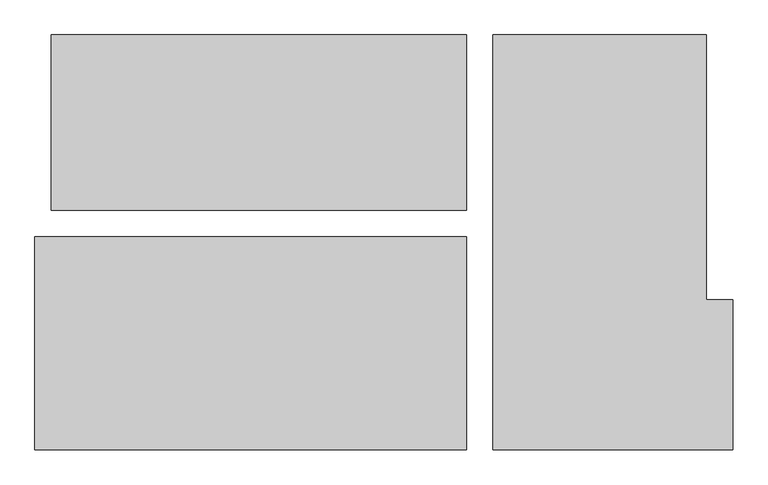
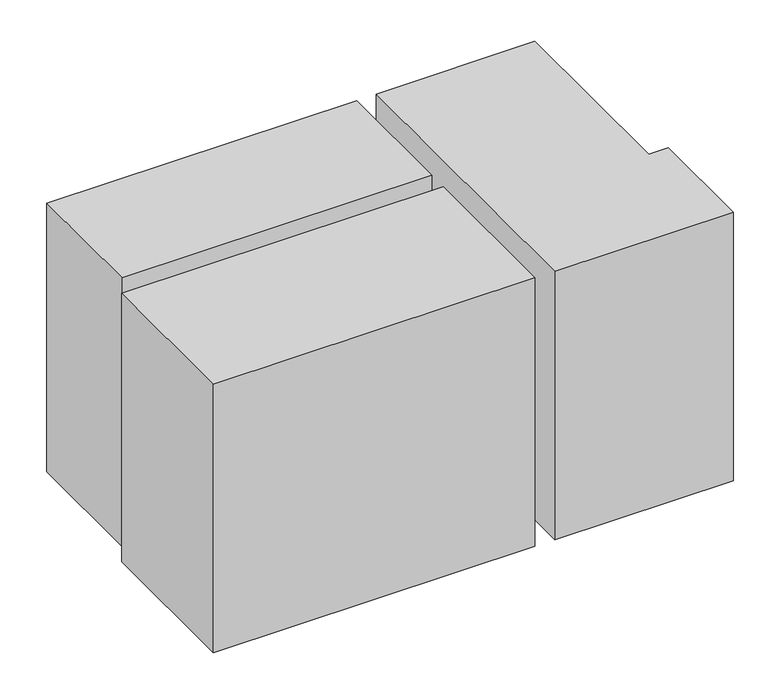
"""IFC4 building model written with IfcOpenShell, lengths in millimetres: proxy geometry, 0_3d."""

from ifc_helpers import new_model, si_unit, origin, origin_with_axes, place, context, project, spatial, polyline, outline, extrude, source, transform, mapped, element, save


def generic_models_d6ef87ce(model_context):
    return source(origin(), model_context, "Body", "SweptSolid", [
        extrude(outline(polyline([(5272.0, 0.0), (3461.9364642, 0.0), (3461.9364642, 3133.4), (5072.0, 3133.4), (5072.0, 1135.0), (5272.0, 1135.0), (5272.0, 0.0)])), origin_with_axes(), (0.0, 0.0, 1.0), 2880.0),
        extrude(outline(polyline([(3261.9364642, 3133.4), (3261.9364642, 1809.3795824), (122.0, 1809.3795824), (122.0, 3133.4), (3261.9364642, 3133.4)])), origin_with_axes(), (0.0, 0.0, 1.0), 2880.0),
        extrude(outline(polyline([(0.0, 1609.3795824), (3261.9364642, 1609.3795824), (3261.9364642, 0.0), (0.0, 0.0), (0.0, 1609.3795824)])), origin_with_axes(), (0.0, 0.0, 1.0), 2880.0),
    ])


if __name__ == "__main__":
    model = new_model("IFC4")
    model_context = context("Model", 3, world=origin())
    ifc_project = project(units=[si_unit("LENGTHUNIT", "METRE", prefix="MILLI")], contexts=[model_context])
    site = spatial("IfcSite", under=ifc_project)
    building = spatial("IfcBuilding", under=site)
    placement = place(None, origin())
    generic_models_shape = generic_models_d6ef87ce(model_context)
    element("IfcBuildingElementProxy", 1, Name="0_3d", ObjectType="0_3d", at=placement, inside=building, context=model_context, shape_type="MappedRepresentation", body=[
        mapped(generic_models_shape, transform((0.0, 0.0, 0.0), x_axis=(1.0, 0.0, 0.0), y_axis=(0.0, 1.0, 0.0), z_axis=(0.0, 0.0, 1.0))),
    ])
    save(model, "model.ifc")

# Revit data of these elements
# Element 1 (IfcBuildingElementProxy, "0_3d")
#   Materials on its faces: "*1"
# Materials
#   "*1": class "Unassigned", colour RGB 175 175 175, transparency 0
